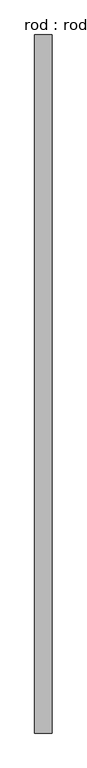
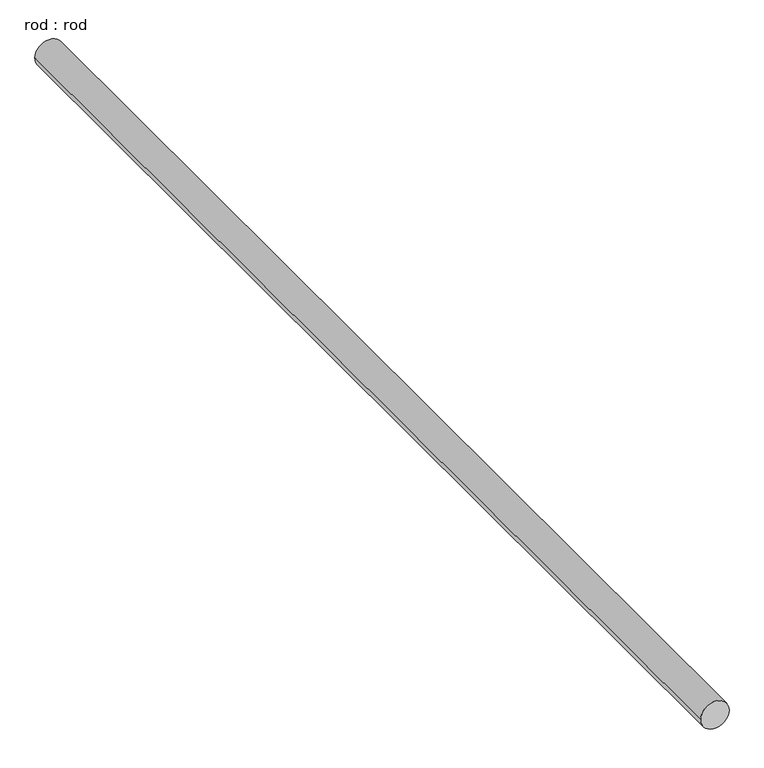
"""IFC4 building model written with IfcOpenShell, lengths in millimetres: proxy geometry, rod : rod."""

from ifc_helpers import new_model, si_unit, point, frame, frame_2d, origin, place, context, project, spatial, circle_curve, trimmed, segment, composite_curve, outline, extrude, source, transform, mapped, element, save


def rod_rod_40cd03c4(model_context):
    return source(origin(), model_context, "Body", "SweptSolid", [
        extrude(outline(composite_curve([segment(trimmed(circle_curve(frame_2d((0.0108462, 0.0)), 200.0), [point((0.0108462, 200.0))], [point((0.0108462, -200.0))], False, "CARTESIAN"), True, "CONTINUOUS"), segment(trimmed(circle_curve(frame_2d((0.0108462, 0.0)), 200.0), [point((0.0108462, -200.0))], [point((0.0108462, 200.0))], False, "CARTESIAN"), True, "CONTINUOUS")], self_intersect=False)), frame((0.0, -3996.5570989, 0.0), z_axis=(0.0, 1.0, 0.0), x_axis=(0.0, 0.0, 1.0)), (0.0, 0.0, 1.0), 16178.5714286),
    ])


if __name__ == "__main__":
    model = new_model("IFC4")
    model_context = context("Model", 3, world=origin())
    ifc_project = project(units=[si_unit("LENGTHUNIT", "METRE", prefix="MILLI")], contexts=[model_context])
    site = spatial("IfcSite", under=ifc_project)
    building = spatial("IfcBuilding", under=site)
    placement = place(None, origin())
    rod_rod_shape = rod_rod_40cd03c4(model_context)
    element("IfcBuildingElementProxy", 1, Name="rod : rod", ObjectType="rod : rod", at=placement, inside=building, context=model_context, shape_type="MappedRepresentation", body=[
        mapped(rod_rod_shape, transform((0.0, 0.0, 0.0), x_axis=(1.0, 0.0, 0.0), y_axis=(0.0, 1.0, 0.0), z_axis=(0.0, 0.0, 1.0))),
    ])
    save(model, "model.ifc")

# Revit data of these elements
# Type "rod : rod"
#   Default Elevation = 0
